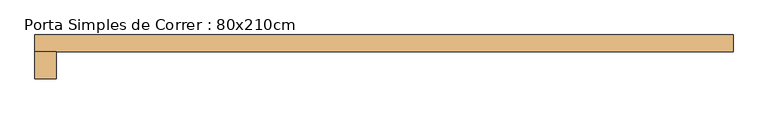
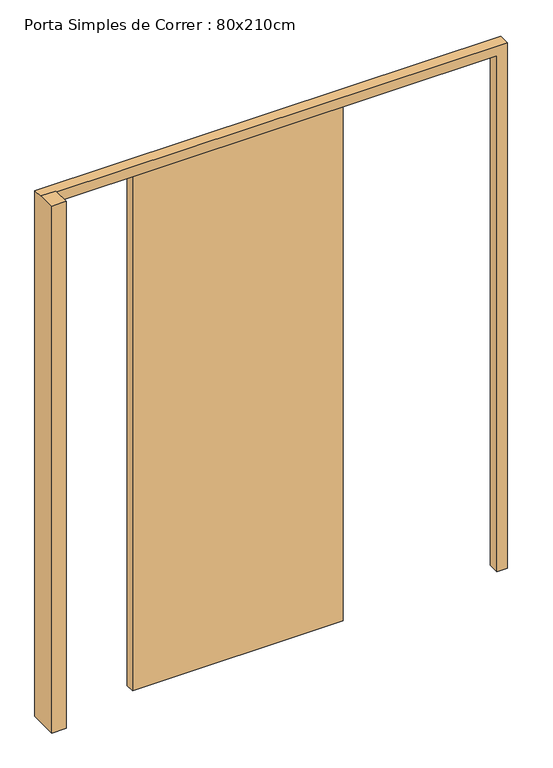
"""IFC4 building model written with IfcOpenShell, lengths in millimetres: door geometry, Porta Simples de Correr : 80x210cm."""

from ifc_helpers import new_model, si_unit, frame, origin, place, context, project, spatial, polyline, outline, extrude, faceted_brep, source, transform, mapped, element, save


def porta_simples_de_correr_80x210cm_4107329d(model_context):
    return source(origin(), model_context, "Body", "SolidModel", [
        extrude(outline(polyline([(814.0, 90.6), (0.0, 90.6), (0.0, 125.6), (814.0, 125.6), (814.0, 90.6)])), frame((0.0, 0.0, 53.0), z_axis=(0.0, 0.0, 1.0), x_axis=(1.0, 0.0, 0.0)), (0.0, 0.0, 1.0), 2099.0),
        faceted_brep([(1445.0, 128.6, 50.0), (1445.0, 85.6, 50.0), (1405.0, 85.6, 50.0), (1405.0, 128.6, 50.0), (1445.0, 128.6, 2195.0), (1445.0, 85.6, 2195.0), (-300.0, 85.6, 2195.0), (-300.0, 85.6, 2155.0), (1405.0, 85.6, 2155.0), (1405.0, 128.6, 2155.0), (-315.0, 128.6, 2155.0), (-315.0, 128.6, 50.0), (-355.0, 128.6, 50.0), (-355.0, 128.6, 2195.0), (-315.0, 85.6, 50.0), (-300.0, 85.6, 50.0), (-300.0, 15.6, 50.0), (-355.0, 15.6, 50.0), (-315.0, 85.6, 2155.0), (-355.0, 15.6, 2200.0), (-355.0, 85.6, 2200.0), (-355.0, 85.6, 2195.0), (-300.0, 85.6, 2200.0), (-300.0, 15.6, 2200.0)], [[[0, 1, 2, 3]], [[1, 0, 4, 5]], [[2, 1, 5, 6, 7, 8]], [[3, 2, 8, 9]], [[0, 3, 9, 10, 11, 12, 13, 4]], [[12, 11, 14, 15, 16, 17]], [[14, 11, 10, 18]], [[12, 17, 19, 20, 21, 13]], [[13, 21, 6, 5, 4]], [[18, 10, 9, 8, 7]], [[16, 15, 7, 6, 22, 23]], [[17, 16, 23, 19]], [[20, 22, 6, 21]], [[15, 14, 18, 7]], [[22, 20, 19, 23]]]),
    ])


if __name__ == "__main__":
    model = new_model("IFC4")
    model_context = context("Model", 3, world=origin())
    ifc_project = project(units=[si_unit("LENGTHUNIT", "METRE", prefix="MILLI")], contexts=[model_context])
    site = spatial("IfcSite", under=ifc_project)
    building = spatial("IfcBuilding", under=site)
    placement = place(None, origin())
    porta_simples_de_correr_80x210cm_shape = porta_simples_de_correr_80x210cm_4107329d(model_context)
    element("IfcDoor", 1, ObjectType="Porta Simples de Correr : 80x210cm", at=placement, inside=building, context=model_context, shape_type="MappedRepresentation", body=[
        mapped(porta_simples_de_correr_80x210cm_shape, transform((0.0, 0.0, 0.0), x_axis=(1.0, 0.0, 0.0), y_axis=(0.0, 1.0, 0.0), z_axis=(0.0, 0.0, 1.0))),
    ])
    save(model, "model.ifc")

# Revit data of these elements
# Type "Porta Simples de Correr : 80x210cm"
#   Type Mark = ""
#   SINAPI = ""
#   Construction Type = "300"
#   Maçaneta [instance default] = ""
#   Fechadura [instance default] = ""
#   Vão Luz (somente para informação) = 80.00 cm
#   Tolerância Folha Vertical = 0.30 cm
#   Módulo Básico M = 10.00 cm
#   Largura de Coordenação Modular Largura CM = 90.00 cm
#   Rough Width = 90.00 cm
#   Deslocamento Horizontal da Folha = 4.00 cm
#   Altura de Coordenação Modular Largura CM = 220.00 cm
#   Rough Height = 220.00 cm
#   Altura Nominal = 209.50 cm
#   Ajuste de Coordenação Topo AC Topo = 0.50 cm
#   Ajuste de Coordenação Base AC Base = 5.00 cm
#   Ajuste de Coordenação AC = 0.00 cm
#   Tolerância Folha Horizontal = 0.30 cm
#   Largura Folha (somente para informação) = 81.40 cm
#   Espessura Folha = 3.50 cm
#   Puxador - Distância da Folha = 5.50 cm
#   Puxador - Altura = 100.00 cm
#   Largura Nominal (Largura Mn) = 82.00 cm
#   Distância do Nível = 0.30 cm
#   Aduela Interna Espessura = 4.00 cm
#   Aduela Interna Comprimento = 7.00 cm
#   Aduela Externa Largura = 180.00 cm
#   Aduela Externa Espessura = 5.00 cm
#   Altura Folha (somente para informação) = 208.90 cm
#   Height = 214.50 cm
#   Width = 90.00 cm
#   Número de Módulos Básicos nM Largura = 9
#   Número de Módulos Básicos nM Altura = 22
#   Batente - Material [instance default] = none
#   Painel - Material [instance default] = none
#   Model = ""
#   Function = (empty or 0)
#   Description = (empty or 0)
#   Wall Closure = (empty or 0)
#   Assembly Code = ""
